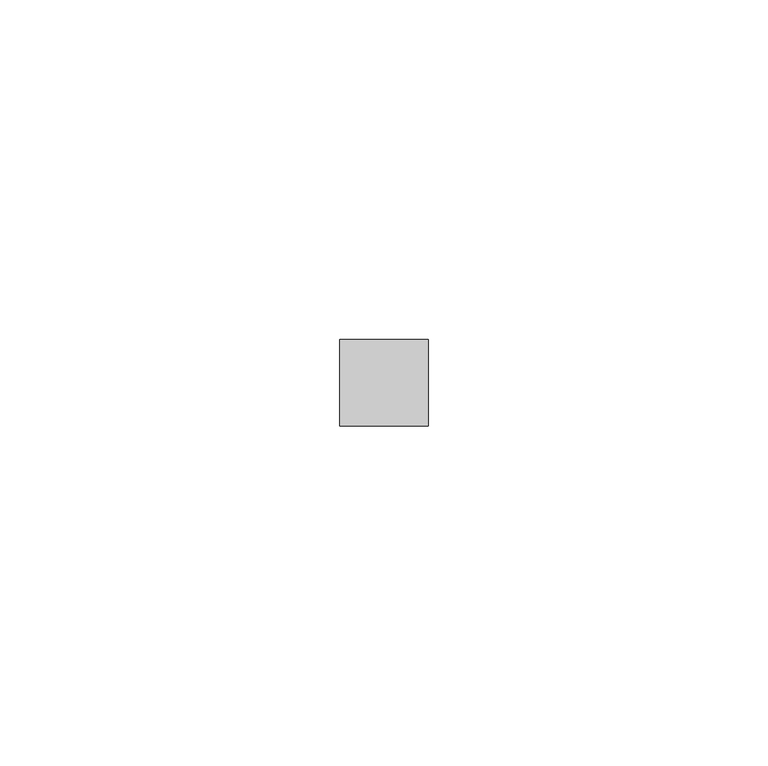
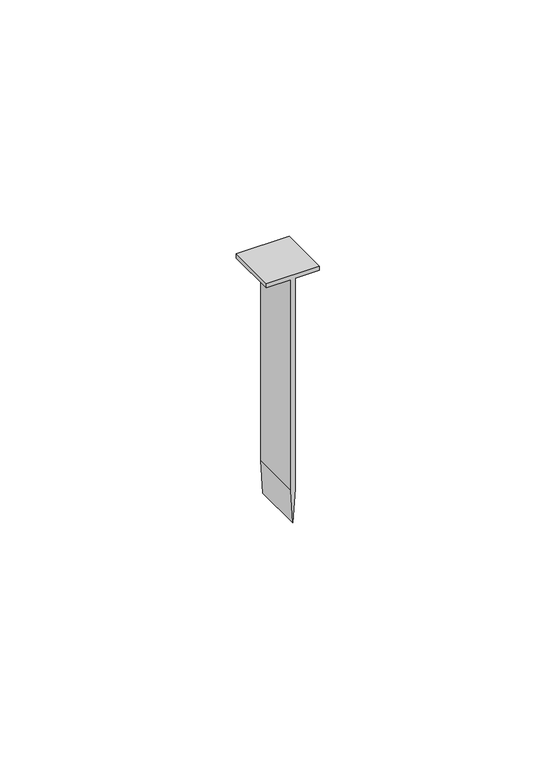
"""IFC4 building model written with IfcOpenShell, lengths in millimetres: proxy geometry, STAINLESS STEEL NAILS010 4139 : STAINLESS STEEL NAILS010 4139."""

from ifc_helpers import new_model, si_unit, frame, origin, place, context, project, spatial, polyline, outline, extrude, source, transform, mapped, element, save


def generic_models_6cd8ff38(model_context):
    return source(origin(), model_context, "Body", "SweptSolid", [
        extrude(outline(polyline([(40259.5998489, -2701.1834531), (40259.5998489, -2695.2258605), (40205.2729558, -2695.2258605), (40196.6073666, -2694.6842611), (40205.2729558, -2694.1426618), (40259.5998489, -2694.1426618), (40259.5998489, -2688.1850692), (40260.6830476, -2688.1850692), (40260.6830476, -2701.1834531), (40259.5998489, -2701.1834531)])), frame((0.0, -1065.5906573, 0.0), z_axis=(0.0, 1.0, 0.0), x_axis=(0.0, 0.0, 1.0)), (0.0, 0.0, 1.0), 12.7),
    ])


if __name__ == "__main__":
    model = new_model("IFC4")
    model_context = context("Model", 3, world=origin())
    ifc_project = project(units=[si_unit("LENGTHUNIT", "METRE", prefix="MILLI")], contexts=[model_context])
    site = spatial("IfcSite", under=ifc_project)
    building = spatial("IfcBuilding", under=site)
    placement = place(None, origin())
    generic_models_shape = generic_models_6cd8ff38(model_context)
    element("IfcBuildingElementProxy", 1, Name="STAINLESS STEEL NAILS010 4139 : STAINLESS STEEL NAILS010 4139", ObjectType="STAINLESS STEEL NAILS010 4139 : STAINLESS STEEL NAILS010 4139", at=placement, inside=building, context=model_context, shape_type="MappedRepresentation", body=[
        mapped(generic_models_shape, transform((0.0, 0.0, 0.0), x_axis=(1.0, 0.0, 0.0), y_axis=(0.0, 1.0, 0.0), z_axis=(0.0, 0.0, 1.0))),
    ])
    save(model, "model.ifc")

# Revit data of these elements
# Type "STAINLESS STEEL NAILS010 4139 : STAINLESS STEEL NAILS010 4139"
#   NameOverride = "STAINLESS STEEL NAILS010"
# Element 1 (IfcBuildingElementProxy, "STAINLESS STEEL NAILS010 4139 : STAINLESS STEEL NAILS010 4139")
#   Materials on its faces: "1 3/4\" STAINLESS STEEL RINGSHANK 5D COMMON NAILS @ 4\" (101.6MM) O.C. FIRESTONE PROVIDED MAX., 1/2\" STAGGERED"
# Materials
#   "1 3/4\" STAINLESS STEEL RINGSHANK 5D COMMON NAILS @ 4\" (101.6MM) O.C. FIRESTONE PROVIDED MAX., 1/2\" STAGGERED": class "Unassigned", colour RGB 255 255 255, transparency 0
